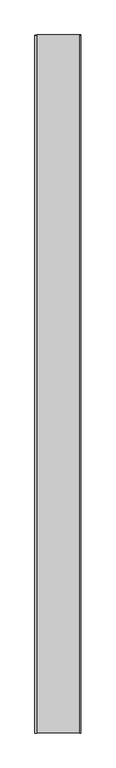
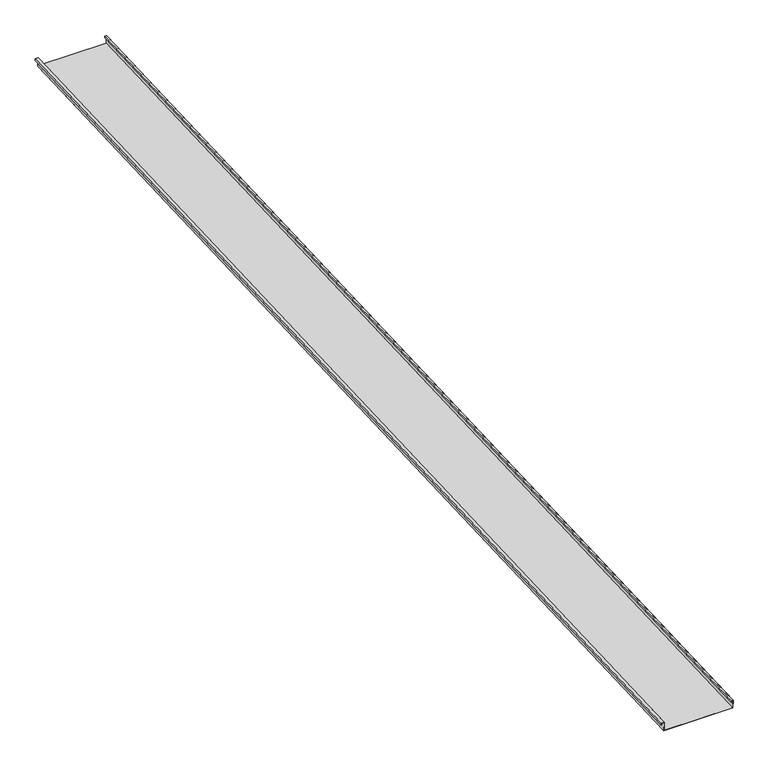
"""IFC4 building model written with IfcOpenShell, lengths in millimetres: proxy geometry, Generic Models 2:Generic Models 2:310765:Generic Models 2:310765 : Generic Models 2:Generic Models 2:310765:111 : Generic Models 2:Generic Models 2:310765:Generic Models 2:310765 : Generic Models 2:Generic Models 2:310765:300385."""

from ifc_helpers import new_model, si_unit, frame, origin, place, context, project, spatial, polyline, outline, extrude, source, transform, mapped, element, save


def generic_models_2eb1153f(model_context):
    return source(origin(), model_context, "Body", "SweptSolid", [
        extrude(outline(polyline([(1.5875, 0.0), (1.5875, 50.8), (407.9875, 50.8), (407.9875, 1.5875), (396.875, 1.5875), (396.875, 11.1125), (398.4625, 11.1125), (398.4625, 3.175), (406.4, 3.175), (406.4, 49.2125), (3.175, 49.2125), (3.175, -1.5874999), (-14.2875, -1.5874999), (-14.2875, 9.525), (-12.7, 9.525), (-12.7, 0.0), (1.5875, 0.0)])), frame((609468.3596406, -581354.4345603, 3902.6697972), z_axis=(0.0, 0.9991330730923568, 0.041630544712067834), x_axis=(1.0, 0.0, 0.0)), (0.0, 0.0, 1.0), 6400.8),
    ])


if __name__ == "__main__":
    model = new_model("IFC4")
    model_context = context("Model", 3, world=origin())
    ifc_project = project(units=[si_unit("LENGTHUNIT", "METRE", prefix="MILLI")], contexts=[model_context])
    site = spatial("IfcSite", under=ifc_project)
    building = spatial("IfcBuilding", under=site)
    placement = place(None, origin())
    generic_models_shape = generic_models_2eb1153f(model_context)
    element("IfcBuildingElementProxy", 1, Name="Generic Models 2:Generic Models 2:310765:Generic Models 2:310765 : Generic Models 2:Generic Models 2:310765:111 : Generic Models 2:Generic Models 2:310765:Generic Models 2:310765 : Generic Models 2:Generic Models 2:310765:300385", ObjectType="Generic Models 2:Generic Models 2:310765:Generic Models 2:310765 : Generic Models 2:Generic Models 2:310765:111 : Generic Models 2:Generic Models 2:310765:Generic Models 2:310765 : Generic Models 2:Generic Models 2:310765:300385", at=placement, inside=building, context=model_context, shape_type="MappedRepresentation", body=[
        mapped(generic_models_shape, transform((0.0, 0.0, 0.0), x_axis=(1.0, 0.0, 0.0), y_axis=(0.0, 1.0, 0.0), z_axis=(0.0, 0.0, 1.0))),
    ])
    save(model, "model.ifc")

# Revit data of these elements
# Type "Generic Models 2:Generic Models 2:310765:Generic Models 2:310765 : Generic Models 2:Generic Models 2:310765:111 : Generic Models 2:Generic Models 2:310765:Generic Models 2:310765 : Generic Models 2:Generic Models 2:310765:300385"
#   NameOverride = "Generic Models 2:Generic Models 2:310765:Generic Models 2:310765 : Generic Models 2:Generic Models 2:310765:300385"
#   ObjectTypeOverride = "Generic Models 2:310765 : Generic Models 2:Generic Models 2:310765"
#   Reference = "Generic Models 2"
#   Tag = "300385"
# Element 1 (IfcBuildingElementProxy, "Generic Models 2:Generic Models 2:310765:Generic Models 2:310765 : Generic Models 2:Generic Models 2:310765:111 : Generic Models 2:Generic Models 2:310765:Generic Models 2:310765 : Generic Models 2:Generic Models 2:310765:300385")
#   Materials on its faces: "THERMAL BROKEN ALUMINUM STOREFRONT FOR POLYCARBONATE"
# Materials
#   "THERMAL BROKEN ALUMINUM STOREFRONT FOR POLYCARBONATE": class "Unassigned", colour RGB 244 244 244, transparency 0, Keynote = "M07611300.01", Cost = 0
